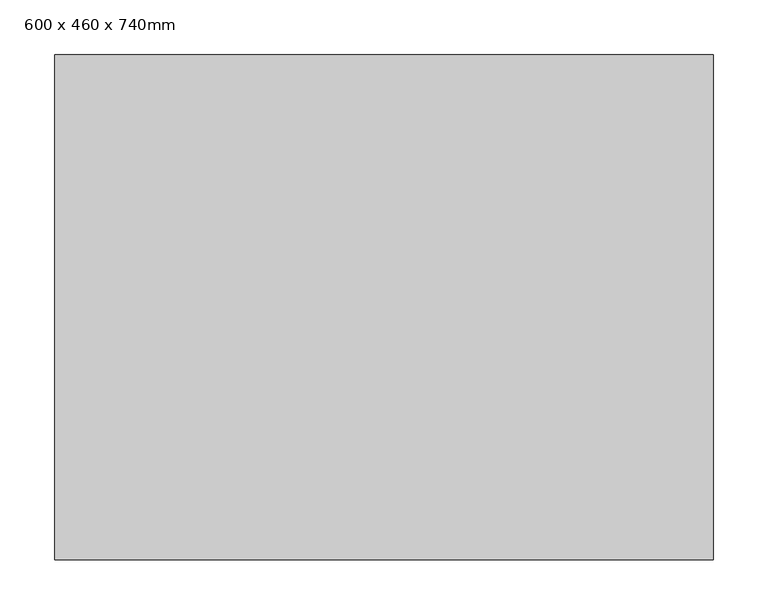
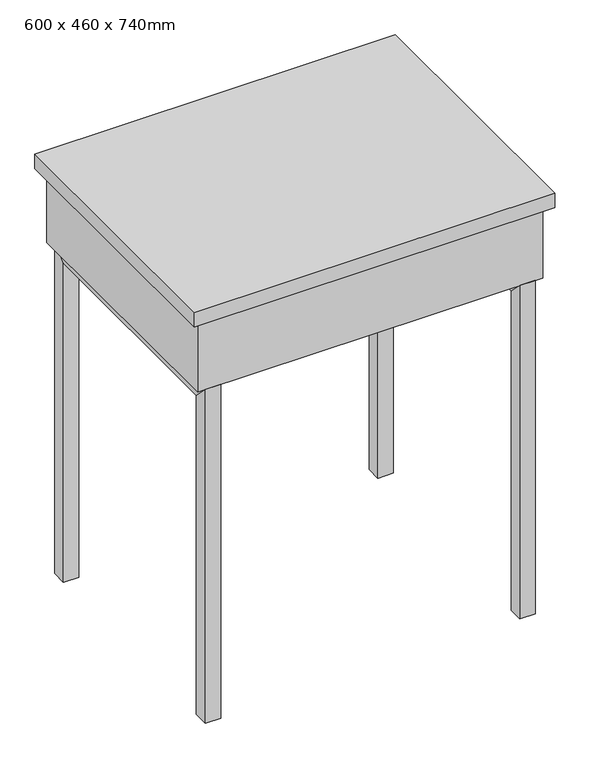
"""IFC4 building model written with IfcOpenShell, lengths in millimetres: furniture geometry, Pult : 600 x 460 x 740mm."""

from ifc_helpers import new_model, si_unit, frame, origin, place, context, project, spatial, polyline, outline, extrude, faceted_brep, source, transform, mapped, element, save


def furniture_600_x_460_x_740mm_67bcbd98(model_context):
    return source(origin(), model_context, "Body", "SolidModel", [
        faceted_brep([(-249.2, -217.3, 0.0), (-274.6, -217.3, 0.0), (-274.6, -191.9, 0.0), (-249.2, -191.9, 0.0), (-249.2, -217.3, 587.6), (-274.6, -217.3, 587.6), (-274.6, -191.9, 562.2), (-249.2, -191.9, 562.2), (-249.2, 217.3, 587.6), (-274.6, 217.3, 587.6), (-274.6, 191.9, 562.2), (-249.2, 191.9, 562.2), (-249.2, 217.3, 0.0), (-249.2, 191.9, 0.0), (-274.6, 191.9, 0.0), (-274.6, 217.3, 0.0)], [[[0, 1, 2, 3]], [[1, 0, 4, 5]], [[2, 1, 5, 6]], [[3, 2, 6, 7]], [[0, 3, 7, 4]], [[5, 4, 8, 9]], [[6, 5, 9, 10]], [[7, 6, 10, 11]], [[4, 7, 11, 8]], [[12, 13, 14, 15]], [[9, 8, 12, 15]], [[10, 9, 15, 14]], [[11, 10, 14, 13]], [[8, 11, 13, 12]]]),
        faceted_brep([(249.2, -217.3, 0.0), (249.2, -191.9, 0.0), (274.6, -191.9, 0.0), (274.6, -217.3, 0.0), (249.2, -217.3, 587.6), (249.2, -191.9, 562.2), (274.6, -191.9, 562.2), (274.6, -217.3, 587.6), (249.2, 217.3, 587.6), (249.2, 191.9, 562.2), (274.6, 191.9, 562.2), (274.6, 217.3, 587.6), (249.2, 217.3, 0.0), (274.6, 217.3, 0.0), (274.6, 191.9, 0.0), (249.2, 191.9, 0.0)], [[[0, 1, 2, 3]], [[1, 0, 4, 5]], [[2, 1, 5, 6]], [[3, 2, 6, 7]], [[0, 3, 7, 4]], [[5, 4, 8, 9]], [[6, 5, 9, 10]], [[7, 6, 10, 11]], [[4, 7, 11, 8]], [[12, 13, 14, 15]], [[9, 8, 12, 15]], [[10, 9, 15, 14]], [[11, 10, 14, 13]], [[8, 11, 13, 12]]]),
        extrude(outline(polyline([(287.3, 217.3), (287.3, -217.3), (-287.3, -217.3), (-287.3, 217.3), (287.3, 217.3)])), frame((0.0, 0.0, 587.6), z_axis=(0.0, 0.0, 1.0), x_axis=(1.0, 0.0, 0.0)), (0.0, 0.0, 1.0), 127.0),
        extrude(outline(polyline([(300.0, 230.0), (300.0, -230.0), (-300.0, -230.0), (-300.0, 230.0), (300.0, 230.0)])), frame((0.0, 0.0, 714.6), z_axis=(0.0, 0.0, 1.0), x_axis=(1.0, 0.0, 0.0)), (0.0, 0.0, 1.0), 25.4),
    ])


if __name__ == "__main__":
    model = new_model("IFC4")
    model_context = context("Model", 3, world=origin())
    ifc_project = project(units=[si_unit("LENGTHUNIT", "METRE", prefix="MILLI")], contexts=[model_context])
    site = spatial("IfcSite", under=ifc_project)
    building = spatial("IfcBuilding", under=site)
    placement = place(None, origin())
    furniture_600_x_460_x_740mm_shape = furniture_600_x_460_x_740mm_67bcbd98(model_context)
    element("IfcFurniture", 1, ObjectType="Pult : 600 x 460 x 740mm", at=placement, inside=building, context=model_context, shape_type="MappedRepresentation", body=[
        mapped(furniture_600_x_460_x_740mm_shape, transform((0.0, 0.0, 0.0), x_axis=(1.0, 0.0, 0.0), y_axis=(0.0, 1.0, 0.0), z_axis=(0.0, 0.0, 1.0))),
    ])
    save(model, "model.ifc")

# Revit data of these elements
# Type "Pult : 600 x 460 x 740mm"
#   Tiefe = 0.460 m
#   Höhe = 0.740 m
#   Breite = 0.600 m
#   Assembly Code = ""
# Element 1 (IfcFurniture, "Pult : 600 x 460 x 740mm")
#   Materials on its faces: "Metall - Chrom", "Metall - Stahl", "Holz - Birke"
# Materials
#   "Metall - Chrom": class "Metall", colour RGB 247 247 247, transparency 0, Cost = 0
#   "Metall - Stahl": class "Metall", colour RGB 247 247 247, transparency 0, Cost = 0
#   "Holz - Birke": class "Holz", colour RGB 213 164 103, transparency 0, Cost = 0
